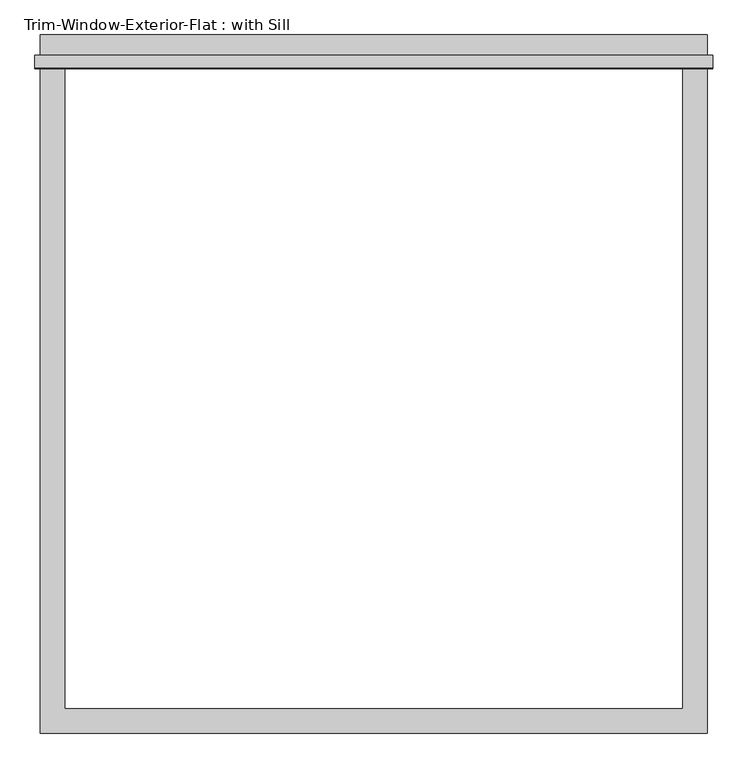
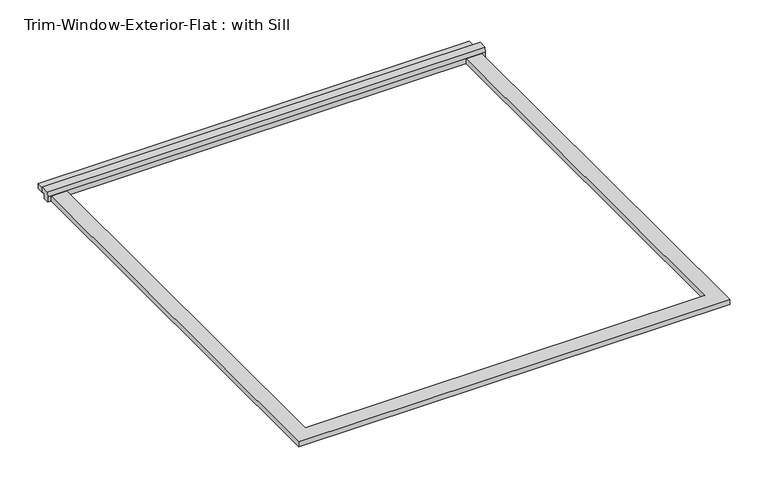
"""IFC4 building model written with IfcOpenShell, lengths in millimetres: proxy geometry, Trim-Window-Exterior-Flat : with Sill."""

from ifc_helpers import new_model, si_unit, frame, origin, origin_with_axes, place, context, project, spatial, polyline, outline, extrude, source, transform, mapped, element, save


def trim_window_exterior_flat_with_sill_d6268ad2(model_context):
    return source(origin(), model_context, "Body", "SweptSolid", [
        extrude(outline(polyline([(781.05, 1520.7823709), (-781.05, 1520.7823709), (-781.05, 1577.9323709), (781.05, 1577.9323709), (781.05, 1520.7823709)])), origin_with_axes(), (0.0, 0.0, 1.0), 19.05),
        extrude(outline(polyline([(1530.35, 38.1), (1530.35, 19.05), (1520.7823709, 19.05), (1520.7823709, 0.0), (1498.6, 0.0), (1498.6, 19.05), (1501.0580645, 38.1), (1530.35, 38.1)])), frame((-793.75, 0.0, 0.0), z_axis=(1.0, 0.0, 0.0), x_axis=(0.0, 1.0, 0.0)), (0.0, 0.0, 1.0), 1587.5),
        extrude(outline(polyline([(-781.05, -57.15), (-781.05, 1498.6), (-723.9, 1498.6), (-723.9, 0.0), (723.9, 0.0), (723.9, 1498.6), (781.05, 1498.6), (781.05, -57.15), (-781.05, -57.15)])), origin_with_axes(), (0.0, 0.0, 1.0), 19.05),
    ])


if __name__ == "__main__":
    model = new_model("IFC4")
    model_context = context("Model", 3, world=origin())
    ifc_project = project(units=[si_unit("LENGTHUNIT", "METRE", prefix="MILLI")], contexts=[model_context])
    site = spatial("IfcSite", under=ifc_project)
    building = spatial("IfcBuilding", under=site)
    placement = place(None, origin())
    trim_window_exterior_flat_with_sill_shape = trim_window_exterior_flat_with_sill_d6268ad2(model_context)
    element("IfcBuildingElementProxy", 1, Name="Trim-Window-Exterior-Flat : with Sill", ObjectType="Trim-Window-Exterior-Flat : with Sill", at=placement, inside=building, context=model_context, shape_type="MappedRepresentation", body=[
        mapped(trim_window_exterior_flat_with_sill_shape, transform((0.0, 0.0, 0.0), x_axis=(1.0, 0.0, 0.0), y_axis=(0.0, 1.0, 0.0), z_axis=(0.0, 0.0, 1.0))),
    ])
    save(model, "model.ifc")

# Revit data of these elements
# Type "Trim-Window-Exterior-Flat : with Sill"
#   Trim Width = 0' - 2 1/4"
#   Trim Thickness_Picture Frame = 0' - 1 1/4"
#   Trim Thickness_with Sill = 0' - 0 3/4"
#   Sill Thickness = 0' - 1 1/4"
#   Opening Width [instance default] = 2' - 0"
#   Opening Height [instance default] = 3' - 0"
#   Default Elevation = 4' - 0"
#   Sill = yes
#   Picture Frame = no
#   Trim Material [instance default] = none
# Element 1 (IfcBuildingElementProxy, "Trim-Window-Exterior-Flat : with Sill")
#   Opening Width = 4' - 9"
#   Opening Height = 4' - 11"
#   Trim Material = Clad - White
#   Materials on its faces: "Clad - White"
# Materials
#   "Clad - White": class "Wood", colour RGB 242 242 238, transparency 0, Cost = 0
